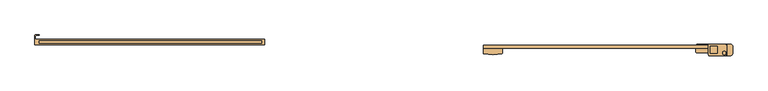
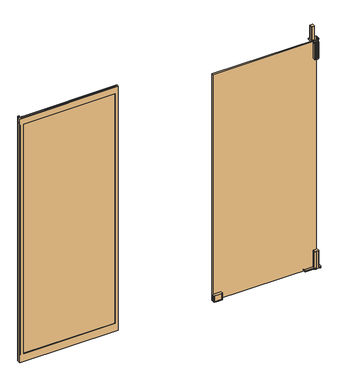
"""IFC4 building model written with IfcOpenShell, lengths in millimetres: door geometry, Otomatik Kapı-Tek Kanat : Otomatik Kapı - Tek Kanat."""

from ifc_helpers import new_model, si_unit, frame, origin, origin_with_axes, place, context, project, spatial, polyline, circle_curve, outline, extrude, source, transform, mapped, element, save
from ifc_brep_helpers import plane_surface, cylinder_surface, revolved_surface, advanced_brep


def door_efeaefdb(model_context):
    return source(origin(), model_context, "Body", "SolidModel", [
        advanced_brep(
        [(-802.5, -155.7669497, 8.0000212), (-799.5330503, -152.8, 8.0000212), (-787.49925, -152.8, 8.0000212), (-787.49925, -154.8, 8.0000212), (-799.4861454, -154.8, 8.0000212), (-800.5, -155.8138546, 8.0000212), (-800.5, -167.3, 8.0000212), (-2.5, -167.3000082, 8.0000212), (-2.5, -187.3, 8.0000212), (-802.5, -187.3, 8.0000212), (-787.49925, -180.7974169, 8.0000212), (-12.4985, -180.7974169, 8.0000212), (-12.4985, -173.8001834, 8.0000212), (-787.49925, -173.8001834, 8.0000212), (-800.5, -167.3, 2101.0), (-800.5, -155.8138546, 2101.0), (-799.4861454, -154.8, 2101.0), (-787.49925, -154.8, 2101.0), (-787.49925, -152.8, 2101.0), (-799.5330503, -152.8, 2101.0), (-802.5, -155.7669497, 2101.0), (-802.5, -187.3, 2101.0), (-2.5, -187.3, 2101.0), (-2.5, -167.3, 2101.0), (-787.49925, -172.299, 2101.0), (-12.4985, -172.299, 2101.0), (-12.4985, -182.301, 2101.0), (-787.49925, -182.301, 2101.0), (-802.5, -187.3, 78.000055), (-802.5, -185.3, 78.000055), (-802.5, -185.3, 62.9982446), (-802.5, -184.239458, 62.9982446), (-802.5, -184.239458, 2061.0007973), (-802.5, -185.3, 2061.0007973), (-802.5, -185.3, 2046.0007973), (-802.5, -187.3, 2046.0007973), (-772.4862373, -167.3, 2046.0004744), (-772.4862373, -169.2993721, 2046.0004744), (-772.4862373, -169.2993721, 77.9999799), (-772.4862373, -167.3, 77.9999799), (-787.49925, -169.2993721, 2061.0007973), (-787.49925, -169.2993721, 62.9982446), (-12.4985, -169.2993721, 62.9982446), (-12.4985, -169.2993721, 2061.0007973), (-27.4985, -169.2993721, 2046.0004744), (-27.4985, -169.2993721, 77.9999799), (-787.49925, -173.8001834, 33.4998483), (-787.49925, -180.7974169, 33.4998483), (-787.49925, -182.301, 2092.5), (-787.49925, -172.299, 2092.5), (-787.49925, -185.3, 2061.0007973), (-787.49925, -185.3, 62.9982446), (-802.3103756, -185.3, 78.000055), (-802.3103756, -185.3, 62.9982446), (-802.3103756, -185.3, 2061.0007973), (-802.3103756, -185.3, 2046.0007973), (-12.4985, -185.3, 2061.0007973), (-12.4985, -185.3, 62.9982446), (-772.4985, -185.3, 2046.0007973), (-772.4985, -185.3, 78.000055), (-27.4985, -185.3, 78.000055), (-27.4985, -185.3, 2046.0007973), (-772.4985, -187.3, 2046.0007973), (-772.4985, -187.3, 78.000055), (-799.439458, -187.3, 2046.0007973), (-799.439458, -187.3, 78.000055), (-27.4985, -187.3, 2046.0007973), (-27.4985, -187.3, 78.000055), (-27.4985, -167.3, 77.9999799), (-27.4985, -167.3, 2046.0004744), (-12.4985, -182.301, 2092.5), (-12.4985, -172.299, 2092.5), (-12.4985, -173.8001834, 33.4998483), (-12.4985, -180.7974169, 33.4998483)],
        [
            (0, 1, circle_curve(frame((-799.5330503, -155.7669497, 8.0000212), z_axis=(0.0, 0.0, -1.0), x_axis=(-1.0, 0.0, 0.0)), 2.9669497)),
            (1, 2),
            (2, 3),
            (3, 4),
            (4, 5, circle_curve(frame((-799.4861454, -155.8138546, 8.0000212), z_axis=(0.0, 0.0, 1.0), x_axis=(-1.0, 0.0, 0.0)), 1.0138546)),
            (5, 6),
            (6, 7),
            (7, 8),
            (8, 9),
            (9, 0),
            (10, 11),
            (11, 12),
            (12, 13),
            (13, 10),
            (14, 15),
            (15, 16, circle_curve(frame((-799.4861454, -155.8138546, 2101.0), z_axis=(0.0, 0.0, -1.0), x_axis=(-1.0, 0.0, 0.0)), 1.0138546)),
            (16, 17),
            (17, 18),
            (18, 19),
            (19, 20, circle_curve(frame((-799.5330503, -155.7669497, 2101.0), z_axis=(0.0, 0.0, 1.0), x_axis=(-1.0, 0.0, 0.0)), 2.9669497)),
            (20, 21),
            (21, 22),
            (22, 23),
            (23, 14),
            (24, 25),
            (25, 26),
            (26, 27),
            (27, 24),
            (20, 0),
            (9, 28),
            (28, 29),
            (29, 30),
            (30, 31),
            (31, 32),
            (32, 33),
            (33, 34),
            (34, 35),
            (35, 21),
            (1, 19),
            (18, 2),
            (17, 3),
            (36, 37),
            (37, 38),
            (38, 39),
            (39, 36),
            (40, 41),
            (41, 42),
            (42, 43),
            (43, 40),
            (37, 44),
            (44, 45),
            (45, 38),
            (13, 46),
            (46, 47),
            (47, 10),
            (27, 48),
            (48, 49),
            (49, 24),
            (40, 50),
            (50, 51),
            (51, 41),
            (29, 52),
            (52, 53),
            (53, 30),
            (33, 54),
            (54, 55),
            (55, 34),
            (50, 56),
            (56, 57),
            (57, 51),
            (58, 59),
            (59, 60),
            (60, 61),
            (61, 58),
            (58, 62),
            (62, 63),
            (63, 59),
            (35, 64),
            (64, 65),
            (65, 28),
            (8, 22),
            (62, 66),
            (66, 67),
            (67, 63),
            (23, 7),
            (6, 14),
            (39, 68),
            (68, 69),
            (69, 36),
            (16, 4),
            (5, 15),
            (54, 32, circle_curve(frame((-799.439458, -184.239458, 2061.0007973), z_axis=(0.0, 0.0, -1.0), x_axis=(-1.0, 0.0, 0.0)), 3.060542)),
            (31, 53, circle_curve(frame((-799.439458, -184.239458, 62.9982446), z_axis=(0.0, 0.0, 1.0), x_axis=(-1.0, 0.0, 0.0)), 3.060542)),
            (52, 65, circle_curve(frame((-799.439458, -184.239458, 78.000055), z_axis=(0.0, 0.0, 1.0), x_axis=(-1.0, 0.0, 0.0)), 3.060542)),
            (64, 55, circle_curve(frame((-799.439458, -184.239458, 2046.0007973), z_axis=(0.0, 0.0, -1.0), x_axis=(-1.0, 0.0, 0.0)), 3.060542)),
            (26, 70),
            (70, 48),
            (70, 71),
            (71, 49),
            (71, 25),
            (69, 44),
            (43, 56),
            (61, 66),
            (67, 60),
            (57, 42),
            (45, 68),
            (12, 72),
            (72, 46),
            (72, 73),
            (73, 47),
            (73, 11),
        ],
        [
            plane_surface(frame((-802.5, -167.3, 8.0000212), z_axis=(0.0, 0.0, -1.0), x_axis=(0.0, -1.0, 0.0))),
            plane_surface(frame((-802.5, -167.3, 2101.0), z_axis=(0.0, 0.0, 1.0), x_axis=(0.0, -1.0, 0.0))),
            plane_surface(frame((-802.5, -184.239458, 8.0000212), z_axis=(-1.0, 0.0, 0.0), x_axis=(0.0, 0.0, 1.0))),
            plane_surface(frame((-799.5330503, -152.8, 8.0000212), z_axis=(0.0, 1.0, 0.0), x_axis=(0.0, 0.0, 1.0))),
            plane_surface(frame((-787.49925, -152.8, 8.0000212), z_axis=(1.0, 0.0, 0.0), x_axis=(0.0, 0.0, 1.0))),
            plane_surface(frame((-772.4862373, -167.3, 8.0000212), z_axis=(1.0, 0.0, 0.0), x_axis=(0.0, 0.0, 1.0))),
            plane_surface(frame((-772.4862373, -169.2993721, 8.0000212), z_axis=(0.0, -1.0, 0.0), x_axis=(0.0, 0.0, 1.0))),
            plane_surface(frame((-787.49925, -169.2993721, 8.0000212), z_axis=(1.0, 0.0, 0.0), x_axis=(0.0, 0.0, 1.0))),
            plane_surface(frame((-787.49925, -185.3, 8.0000212), z_axis=(0.0, 1.0, 0.0), x_axis=(0.0, 0.0, 1.0))),
            plane_surface(frame((-772.4985, -185.3, 8.0000212), z_axis=(1.0, 0.0, 0.0), x_axis=(0.0, 0.0, 1.0))),
            plane_surface(frame((-772.4985, -187.3, 8.0000212), z_axis=(0.0, -1.0, 0.0), x_axis=(0.0, 0.0, 1.0))),
            plane_surface(frame((-800.5, -167.3, 8.0000212), z_axis=(0.0, 1.0, 0.0), x_axis=(0.0, 0.0, 1.0))),
            plane_surface(frame((-787.49925, -154.8, 8.0000212), z_axis=(0.0, -1.0, 0.0), x_axis=(0.0, 0.0, 1.0))),
            plane_surface(frame((-800.5, -155.8138546, 8.0000212), z_axis=(1.0, 0.0, 0.0), x_axis=(0.0, 0.0, 1.0))),
            cylinder_surface(frame((-799.439458, -184.239458, 8.0000212), z_axis=(0.0, 0.0, -1.0), x_axis=(-1.0, 0.0, 0.0)), 3.060542),
            cylinder_surface(frame((-799.5330503, -155.7669497, 8.0000212), z_axis=(0.0, 0.0, -1.0), x_axis=(-1.0, 0.0, 0.0)), 2.9669497),
            revolved_surface(polyline([(-800.5, -155.8138546, 2101.0), (-800.5, -155.8138546, 8.0000212)]), (-799.4861454, -155.8138546, 8.0000212), (0.0, 0.0, 1.0)),
            plane_surface(frame((-2.5, -167.3, 2101.0), z_axis=(1.0, 0.0, 0.0), x_axis=(0.0, -1.0, 0.0))),
            plane_surface(frame((-802.5, -182.301, 2101.0), z_axis=(0.0, 1.0, 0.0), x_axis=(1.0, 0.0, 0.0))),
            plane_surface(frame((-802.5, -182.301, 2092.5), z_axis=(0.0, 0.0, 1.0), x_axis=(1.0, 0.0, 0.0))),
            plane_surface(frame((-802.5, -172.299, 2092.5), z_axis=(0.0, -1.0, 0.0), x_axis=(1.0, 0.0, 0.0))),
            plane_surface(frame((-802.5, -167.3, 2046.0004744), z_axis=(0.0, 0.0, -1.0), x_axis=(1.0, 0.0, 0.0))),
            plane_surface(frame((-802.5, -169.3, 2061.0007973), z_axis=(0.0, 0.0, -1.0), x_axis=(1.0, 0.0, 0.0))),
            plane_surface(frame((-802.5, -185.3, 2046.0007973), z_axis=(0.0, 0.0, -1.0), x_axis=(1.0, 0.0, 0.0))),
            plane_surface(frame((-802.5, -187.3, 78.000055), z_axis=(0.0, 0.0, 1.0), x_axis=(1.0, 0.0, 0.0))),
            plane_surface(frame((-802.5, -185.3, 62.9982446), z_axis=(0.0, 0.0, 1.0), x_axis=(1.0, 0.0, 0.0))),
            plane_surface(frame((-802.5, -169.3000224, 77.9999799), z_axis=(0.0, 0.0, 1.0), x_axis=(1.0, 0.0, 0.0))),
            plane_surface(frame((-802.5, -173.8001834, 8.0000212), z_axis=(0.0, -1.0, 0.0), x_axis=(1.0, 0.0, 0.0))),
            plane_surface(frame((-802.5, -173.8001834, 33.4998483), z_axis=(0.0, 0.0, -1.0), x_axis=(1.0, 0.0, 0.0))),
            plane_surface(frame((-802.5, -180.7974169, 33.4998483), z_axis=(0.0, 1.0, 0.0), x_axis=(1.0, 0.0, 0.0))),
            plane_surface(frame((-27.4985, -187.3, 8.0000212), z_axis=(-1.0, 0.0, 0.0), x_axis=(0.0, 0.0, 1.0))),
            plane_surface(frame((-12.4985, -185.3, 8.0000212), z_axis=(-1.0, 0.0, 0.0), x_axis=(0.0, 0.0, 1.0))),
            plane_surface(frame((-27.4985, -169.3, 8.0000212), z_axis=(-1.0, 0.0, 0.0), x_axis=(0.0, 0.0, 1.0))),
        ],
        [
            (0, [[1, 2, 3, 4, 5, 6, 7, 8, 9, 10], [11, 12, 13, 14]]),
            (1, [[15, 16, 17, 18, 19, 20, 21, 22, 23, 24], [25, 26, 27, 28]]),
            (2, [[29, -10, 30, 31, 32, 33, 34, 35, 36, 37, 38, -21]]),
            (3, [[-2, 39, -19, 40]]),
            (4, [[-3, -40, -18, 41]]),
            (5, [[42, 43, 44, 45]]),
            (6, [[46, 47, 48, 49], [-43, 50, 51, 52]]),
            (7, [[-14, 53, 54, 55]]),
            (7, [[-28, 56, 57, 58]]),
            (7, [[59, 60, 61, -46]]),
            (8, [[-32, 62, 63, 64]]),
            (8, [[-36, 65, 66, 67]]),
            (8, [[-60, 68, 69, 70], [71, 72, 73, 74]]),
            (9, [[75, 76, 77, -71]]),
            (10, [[-22, -38, 78, 79, 80, -30, -9, 81], [82, 83, 84, -76]]),
            (11, [[-24, 85, -7, 86], [87, 88, 89, -45]]),
            (12, [[-4, -41, -17, 90]]),
            (13, [[-6, 91, -15, -86]]),
            (14, [[92, -34, 93, -63, 94, -79, 95, -66]]),
            (15, [[-1, -29, -20, -39]]),
            (16, [[-5, -90, -16, -91]]),
            (17, [[-81, -8, -85, -23]]),
            (18, [[-56, -27, 96, 97]]),
            (19, [[-57, -97, 98, 99]]),
            (20, [[-58, -99, 100, -25]]),
            (21, [[-42, -89, 101, -50]]),
            (22, [[-35, -92, -65]]),
            (22, [[-68, -59, -49, 102]]),
            (23, [[-37, -67, -95, -78]]),
            (23, [[-75, -74, 103, -82]]),
            (24, [[-31, -80, -94, -62]]),
            (24, [[-77, -84, 104, -72]]),
            (25, [[-33, -64, -93]]),
            (25, [[-47, -61, -70, 105]]),
            (26, [[-44, -52, 106, -87]]),
            (27, [[-53, -13, 107, 108]]),
            (28, [[-54, -108, 109, 110]]),
            (29, [[-55, -110, 111, -11]]),
            (30, [[-73, -104, -83, -103]]),
            (31, [[-12, -111, -109, -107]]),
            (31, [[-26, -100, -98, -96]]),
            (31, [[-69, -102, -48, -105]]),
            (32, [[-88, -106, -51, -101]]),
        ],
    ),
        extrude(outline(polyline([(-14.9985, -170.3000147), (-14.9985, -180.2993696), (-784.0, -180.2993696), (-784.0, -170.3000147), (-14.9985, -170.3000147)])), frame((0.0, 0.0, 65.4907153), z_axis=(0.0, 0.0, 1.0), x_axis=(1.0, 0.0, 0.0)), (0.0, 0.0, 1.0), 1993.010082),
        extrude(outline(polyline([(-170.3000393, 2058.9584681), (-170.3000367, 2075.4578872), (-169.3000368, 2075.4578872), (-169.3000392, 2060.1996761), (-167.7000392, 2060.1994116), (-167.7000392, 2059.1856312), (-170.3000393, 2058.9584681)])), frame((-802.5, 0.0, 0.0), z_axis=(1.0, 0.0, 0.0), x_axis=(0.0, 1.0, 0.0)), (0.0, 0.0, 1.0), 800.0),
        extrude(outline(polyline([(-170.3000147, 79.2411881), (-167.7000146, 79.0140251), (-167.7000146, 78.0002446), (-169.3000145, 77.9999802), (-169.3000145, 62.7412326), (-170.3000121, 62.7417691), (-170.3000147, 79.2411881)])), frame((-802.5, 0.0, 0.0), z_axis=(1.0, 0.0, 0.0), x_axis=(0.0, 1.0, 0.0)), (0.0, 0.0, 1.0), 800.0),
        extrude(outline(polyline([(-783.1860852, -169.2999998), (-772.5, -169.2999998), (-772.5, -167.6999998), (-771.385912, -167.6999998), (-771.0906874, -170.50022), (-783.1860852, -170.50022), (-783.1860852, -169.2999998)])), frame((0.0, 0.0, 8.0000212), z_axis=(0.0, 0.0, 1.0), x_axis=(1.0, 0.0, 0.0)), (0.0, 0.0, 1.0), 2092.9999788),
        advanced_brep(
        [(1574.3473639, -189.1450647, 150.5), (1599.9937802, -189.1450647, 150.5), (1599.9937802, -199.1283088, 150.5), (1574.9937802, -199.1283088, 150.5), (1574.9937802, -217.3610561, 150.5), (1587.4005623, -224.1450647, 150.5), (1605.2100763, -224.1450647, 150.5), (1606.9937802, -222.3613608, 150.5), (1606.9937802, -187.0776187, 150.5), (1605.0612263, -185.1450647, 150.5), (1576.2799178, -185.1450647, 150.5), (1574.3473639, -187.0776187, 150.5), (1578.9203726, -221.1098306, 8.0), (1574.9937802, -217.3610561, 8.0), (1577.1630779, -219.3712473, 8.0), (1574.3473639, -189.1450647, 8.0), (1599.9937802, -189.1450647, 8.0), (1599.9937802, -199.1283088, 8.0), (1574.9937802, -199.1283088, 8.0), (1587.4005623, -224.1450647, 8.0), (1587.4005623, -224.1450647, 0.0), (1619.8416735, -224.1450647, 0.0), (1619.8416735, -224.1450647, 8.0), (1605.2100763, -224.1450647, 8.0), (1606.9937802, -222.3613608, 8.0), (1606.9937802, -187.0776187, 8.0), (1605.0612263, -185.1450647, 8.0), (1619.9440671, -185.1450647, 8.0), (1619.9440671, -185.1450647, 0.0), (1504.0, -185.1450647, 0.0), (1504.0, -185.1450647, 8.0), (1576.2799178, -185.1450647, 8.0), (1574.3473639, -187.0776187, 8.0), (1627.0, -192.2009976, 0.0), (1627.0, -216.9867382, 0.0), (1577.1630779, -219.3712473, 0.0), (1568.1, -215.1450647, 0.0), (1504.0, -215.1450647, 0.0), (1499.0, -210.1450647, 0.0), (1499.0, -190.1450647, 0.0), (1627.0, -216.9867382, 8.0), (1627.0, -192.2009976, 8.0), (1499.0, -190.1450647, 8.0), (1499.0, -210.1450647, 8.0), (1504.0, -215.1450647, 8.0), (1568.1, -215.1450647, 8.0)],
        [
            (0, 1),
            (1, 2),
            (2, 3),
            (3, 4),
            (4, 5, circle_curve(frame((1588.8230743, -206.8065986, 150.5), z_axis=(0.0, 0.0, 1.0), x_axis=(-1.0, 0.0, 0.0)), 17.3967223)),
            (5, 6),
            (6, 7, circle_curve(frame((1605.2100763, -222.3613608, 150.5), z_axis=(0.0, 0.0, 1.0), x_axis=(-1.0, 0.0, 0.0)), 1.7837039)),
            (7, 8),
            (8, 9, circle_curve(frame((1605.0612263, -187.0776187, 150.5), z_axis=(0.0, 0.0, 1.0), x_axis=(-1.0, 0.0, 0.0)), 1.932554)),
            (9, 10),
            (10, 11, circle_curve(frame((1576.2799178, -187.0776187, 150.5), z_axis=(0.0, 0.0, 1.0), x_axis=(-1.0, 0.0, 0.0)), 1.932554)),
            (11, 0),
            (12, 13, circle_curve(frame((1588.8230743, -206.8065986, 8.0), z_axis=(0.0, 0.0, -1.0), x_axis=(-1.0, 0.0, 0.0)), 17.3967223)),
            (13, 14, circle_curve(frame((1568.1, -226.9760726, 8.0), z_axis=(0.0, 0.0, -1.0), x_axis=(-1.0, 0.0, 0.0)), 11.8310079)),
            (14, 12, circle_curve(frame((1587.4005623, -210.7809779, 8.0), z_axis=(0.0, 0.0, 1.0), x_axis=(-1.0, 0.0, 0.0)), 13.3640868)),
            (0, 15),
            (15, 16),
            (16, 1),
            (16, 17),
            (17, 2),
            (17, 18),
            (18, 3),
            (18, 13),
            (13, 4),
            (12, 19, circle_curve(frame((1588.8230743, -206.8065986, 8.0), z_axis=(0.0, 0.0, 1.0), x_axis=(-1.0, 0.0, 0.0)), 17.3967223)),
            (19, 5),
            (19, 20),
            (20, 21),
            (21, 22),
            (22, 23),
            (23, 6),
            (23, 24, circle_curve(frame((1605.2100763, -222.3613608, 8.0), z_axis=(0.0, 0.0, 1.0), x_axis=(-1.0, 0.0, 0.0)), 1.7837039)),
            (24, 7),
            (24, 25),
            (25, 8),
            (25, 26, circle_curve(frame((1605.0612263, -187.0776187, 8.0), z_axis=(0.0, 0.0, 1.0), x_axis=(-1.0, 0.0, 0.0)), 1.932554)),
            (26, 9),
            (26, 27),
            (27, 28),
            (28, 29),
            (29, 30),
            (30, 31),
            (31, 10),
            (31, 32, circle_curve(frame((1576.2799178, -187.0776187, 8.0), z_axis=(0.0, 0.0, 1.0), x_axis=(-1.0, 0.0, 0.0)), 1.932554)),
            (32, 11),
            (32, 15),
            (28, 33, circle_curve(frame((1619.9440671, -192.2009976, 0.0), z_axis=(0.0, 0.0, -1.0), x_axis=(-1.0, 0.0, 0.0)), 7.0559329)),
            (33, 34),
            (34, 21, circle_curve(frame((1619.8416735, -216.9867382, 0.0), z_axis=(0.0, 0.0, -1.0), x_axis=(-1.0, 0.0, 0.0)), 7.1583265)),
            (20, 35, circle_curve(frame((1587.4005623, -210.7809779, 0.0), z_axis=(0.0, 0.0, -1.0), x_axis=(-1.0, 0.0, 0.0)), 13.3640868)),
            (35, 36, circle_curve(frame((1568.1, -226.9760726, 0.0), z_axis=(0.0, 0.0, 1.0), x_axis=(-1.0, 0.0, 0.0)), 11.8310079)),
            (36, 37),
            (37, 38, circle_curve(frame((1504.0, -210.1450647, 0.0), z_axis=(0.0, 0.0, -1.0), x_axis=(-1.0, 0.0, 0.0)), 5.0)),
            (38, 39),
            (39, 29, circle_curve(frame((1504.0, -190.1450647, 0.0), z_axis=(0.0, 0.0, -1.0), x_axis=(-1.0, 0.0, 0.0)), 5.0)),
            (12, 19, circle_curve(frame((1587.4005623, -210.7809779, 8.0), z_axis=(0.0, 0.0, 1.0), x_axis=(-1.0, 0.0, 0.0)), 13.3640868)),
            (22, 40, circle_curve(frame((1619.8416735, -216.9867382, 8.0), z_axis=(0.0, 0.0, 1.0), x_axis=(-1.0, 0.0, 0.0)), 7.1583265)),
            (40, 41),
            (41, 27, circle_curve(frame((1619.9440671, -192.2009976, 8.0), z_axis=(0.0, 0.0, 1.0), x_axis=(-1.0, 0.0, 0.0)), 7.0559329)),
            (30, 42, circle_curve(frame((1504.0, -190.1450647, 8.0), z_axis=(0.0, 0.0, 1.0), x_axis=(-1.0, 0.0, 0.0)), 5.0)),
            (42, 43),
            (43, 44, circle_curve(frame((1504.0, -210.1450647, 8.0), z_axis=(0.0, 0.0, 1.0), x_axis=(-1.0, 0.0, 0.0)), 5.0)),
            (44, 45),
            (45, 13, circle_curve(frame((1568.1, -226.9760726, 8.0), z_axis=(0.0, 0.0, -1.0), x_axis=(-1.0, 0.0, 0.0)), 11.8310079)),
            (41, 33),
            (40, 34),
            (14, 35),
            (45, 36),
            (44, 37),
            (43, 38),
            (42, 39),
        ],
        [
            plane_surface(frame((1627.0, -185.1450647, 150.5), z_axis=(0.0, 0.0, 1.0), x_axis=(0.0, 1.0, 0.0))),
            plane_surface(frame((1627.0, -185.1450647, 8.0), z_axis=(0.0, 0.0, -1.0), x_axis=(0.0, 1.0, 0.0))),
            plane_surface(frame((1574.3473639, -189.1450647, 150.5), z_axis=(0.0, -1.0, 0.0), x_axis=(0.0, 0.0, -1.0))),
            plane_surface(frame((1599.9937802, -189.1450647, 150.5), z_axis=(-1.0, 0.0, 0.0), x_axis=(0.0, 0.0, -1.0))),
            plane_surface(frame((1599.9937802, -199.1283088, 150.5), z_axis=(0.0, 1.0, 0.0), x_axis=(0.0, 0.0, -1.0))),
            plane_surface(frame((1574.9937802, -199.1283088, 150.5), z_axis=(-1.0, 0.0, 0.0), x_axis=(0.0, 0.0, -1.0))),
            cylinder_surface(frame((1588.8230743, -206.8065986, 150.5), z_axis=(0.0, 0.0, 1.0), x_axis=(-1.0, 0.0, 0.0)), 17.3967223),
            plane_surface(frame((1587.4005623, -224.1450647, 150.5), z_axis=(0.0, -1.0, 0.0), x_axis=(0.0, 0.0, -1.0))),
            cylinder_surface(frame((1605.2100763, -222.3613608, 150.5), z_axis=(0.0, 0.0, 1.0), x_axis=(-1.0, 0.0, 0.0)), 1.7837039),
            plane_surface(frame((1606.9937802, -222.3613608, 150.5), z_axis=(1.0, 0.0, 0.0), x_axis=(0.0, 0.0, -1.0))),
            cylinder_surface(frame((1605.0612263, -187.0776187, 150.5), z_axis=(0.0, 0.0, 1.0), x_axis=(-1.0, 0.0, 0.0)), 1.932554),
            plane_surface(frame((1605.0612263, -185.1450647, 150.5), z_axis=(0.0, 1.0, 0.0), x_axis=(0.0, 0.0, -1.0))),
            cylinder_surface(frame((1576.2799178, -187.0776187, 150.5), z_axis=(0.0, 0.0, 1.0), x_axis=(-1.0, 0.0, 0.0)), 1.932554),
            plane_surface(frame((1574.3473639, -187.0776187, 150.5), z_axis=(-1.0, 0.0, 0.0), x_axis=(0.0, 0.0, -1.0))),
            plane_surface(frame((1627.0, -185.1450647, 0.0), z_axis=(0.0, 0.0, -1.0), x_axis=(0.0, 1.0, 0.0))),
            plane_surface(frame((1627.0, -185.1450647, 8.0), z_axis=(0.0, 0.0, 1.0), x_axis=(0.0, 1.0, 0.0))),
            cylinder_surface(frame((1619.9440671, -192.2009976, 0.0), z_axis=(0.0, 0.0, -1.0), x_axis=(-1.0, 0.0, 0.0)), 7.0559329),
            plane_surface(frame((1627.0, -192.2009976, 0.0), z_axis=(1.0, 0.0, 0.0), x_axis=(0.0, 0.0, 1.0))),
            cylinder_surface(frame((1619.8416735, -216.9867382, 0.0), z_axis=(0.0, 0.0, -1.0), x_axis=(-1.0, 0.0, 0.0)), 7.1583265),
            cylinder_surface(frame((1587.4005623, -210.7809779, 0.0), z_axis=(0.0, 0.0, -1.0), x_axis=(-1.0, 0.0, 0.0)), 13.3640868),
            revolved_surface(polyline([(1556.2689920999999, -226.9760726, 8.0), (1556.2689920999999, -226.9760726, 0.0)]), (1568.1, -226.9760726, 0.0), (0.0, 0.0, 1.0)),
            plane_surface(frame((1568.1, -215.1450647, 0.0), z_axis=(0.0, -1.0, 0.0), x_axis=(0.0, 0.0, 1.0))),
            cylinder_surface(frame((1504.0, -210.1450647, 0.0), z_axis=(0.0, 0.0, -1.0), x_axis=(-1.0, 0.0, 0.0)), 5.0),
            plane_surface(frame((1499.0, -210.1450647, 0.0), z_axis=(-1.0, 0.0, 0.0), x_axis=(0.0, 0.0, 1.0))),
            cylinder_surface(frame((1504.0, -190.1450647, 0.0), z_axis=(0.0, 0.0, -1.0), x_axis=(-1.0, 0.0, 0.0)), 5.0),
        ],
        [
            (0, [[1, 2, 3, 4, 5, 6, 7, 8, 9, 10, 11, 12]]),
            (1, [[13, 14, 15]]),
            (2, [[-1, 16, 17, 18]]),
            (3, [[-2, -18, 19, 20]]),
            (4, [[-3, -20, 21, 22]]),
            (5, [[-4, -22, 23, 24]]),
            (6, [[-5, -24, -13, 25, 26]]),
            (7, [[-6, -26, 27, 28, 29, 30, 31]]),
            (8, [[-7, -31, 32, 33]]),
            (9, [[-8, -33, 34, 35]]),
            (10, [[-9, -35, 36, 37]]),
            (11, [[-10, -37, 38, 39, 40, 41, 42, 43]]),
            (12, [[-11, -43, 44, 45]]),
            (13, [[-12, -45, 46, -16]]),
            (14, [[-40, 47, 48, 49, -28, 50, 51, 52, 53, 54, 55]]),
            (15, [[56, -25]]),
            (15, [[57, 58, 59, -38, -36, -34, -32, -30]]),
            (15, [[60, 61, 62, 63, 64, -23, -21, -19, -17, -46, -44, -42]]),
            (16, [[-47, -39, -59, 65]]),
            (17, [[-48, -65, -58, 66]]),
            (18, [[-49, -66, -57, -29]]),
            (19, [[-50, -27, -56, -15, 67]]),
            (20, [[-51, -67, -14, -64, 68]]),
            (21, [[-52, -68, -63, 69]]),
            (22, [[-53, -69, -62, 70]]),
            (23, [[-54, -70, -61, 71]]),
            (24, [[-55, -71, -60, -41]]),
        ],
    ),
        advanced_brep(
        [(1572.1438552, -192.4241594, 2085.0), (1550.8144257, -192.4241594, 2085.0), (1548.9791404, -194.2594446, 2085.0), (1548.9791404, -215.5888742, 2085.0), (1550.8144257, -217.4241594, 2085.0), (1572.1438552, -217.4241594, 2085.0), (1573.9791404, -215.5888742, 2085.0), (1573.9791404, -194.2594446, 2085.0), (1572.1438552, -192.4241594, 1970.0), (1550.8144257, -192.4241594, 1970.0), (1548.9791404, -194.2594446, 1970.0), (1548.9791404, -215.5888742, 1970.0), (1550.8144257, -217.4241594, 1970.0), (1572.1438552, -217.4241594, 1970.0), (1573.9791404, -215.5888742, 1970.0), (1573.9791404, -194.2594446, 1970.0), (1545.9964024, -185.1450647, 1970.0), (1542.9937802, -188.1476868, 1970.0), (1542.9937802, -221.823489, 1970.0), (1546.3153559, -225.1450647, 1970.0), (1597.9937802, -225.1450647, 1970.0), (1606.9937802, -216.1450647, 1970.0), (1606.9937802, -193.9739051, 1970.0), (1598.1649399, -185.1450647, 1970.0), (1597.9937802, -222.0450647, 1970.0), (1597.9937802, -210.2450647, 1970.0), (1545.9964024, -185.1450647, 1964.0), (1598.1649399, -185.1450647, 1964.0), (1606.9937802, -193.9739051, 1964.0), (1606.9937802, -216.1450647, 1964.0), (1597.9937802, -225.1450647, 1964.0), (1546.3153559, -225.1450647, 1964.0), (1542.9937802, -221.823489, 1964.0), (1542.9937802, -188.1476868, 1964.0), (1597.9937802, -210.2450647, 1964.0), (1597.9937802, -222.0450647, 1964.0), (1606.9937802, -216.1450647, 1798.2), (1591.4461955, -222.319944, 1798.2), (1587.411505, -225.1450647, 1798.2), (1578.0937802, -225.1450647, 1798.2), (1574.9937802, -222.0450647, 1798.2), (1574.9937802, -199.2450647, 1798.2), (1599.7937802, -199.2450647, 1798.2), (1599.7937802, -189.2450647, 1798.2), (1574.9937802, -189.2450647, 1798.2), (1574.9937802, -186.4710526, 1798.2), (1576.3197681, -185.1450647, 1798.2), (1605.7821796, -185.1450647, 1798.2), (1606.9937802, -186.3566653, 1798.2), (1587.2194224, -210.2450647, 1798.2), (1578.0937802, -210.2450647, 1798.2), (1578.0937802, -221.0562868, 1798.2), (1579.0825581, -222.0450647, 1798.2), (1587.1673699, -222.0450647, 1798.2), (1588.942968, -219.8725331, 1798.2), (1588.9937802, -212.0194225, 1798.2), (1597.9937802, -210.2450647, 1798.2), (1597.9937802, -222.0450647, 1798.2), (1606.9937802, -216.1450647, 1943.2), (1606.9937802, -186.3566653, 1943.2), (1605.7821796, -185.1450647, 1943.2), (1576.3197681, -185.1450647, 1943.2), (1574.9937802, -186.4710526, 1943.2), (1574.9937802, -189.2450647, 1943.2), (1599.7937802, -189.2450647, 1943.2), (1599.7937802, -199.2450647, 1943.2), (1574.9937802, -199.2450647, 1943.2), (1574.9937802, -209.0670845, 1943.2), (1576.1717604, -210.2450647, 1943.2), (1587.2194224, -210.2450647, 1943.2), (1588.9937802, -212.0194225, 1943.2), (1588.9937802, -216.1450647, 1943.2), (1597.9937802, -222.0450647, 1943.2), (1597.9937802, -210.2450647, 1943.2), (1574.9937802, -222.0450647, 1933.2), (1574.9937802, -209.0670845, 1933.2), (1576.1717604, -210.2450647, 1933.2), (1578.0937802, -210.2450647, 1933.2), (1588.9937802, -219.8725331, 1933.2), (1588.9937802, -216.1450647, 1933.2), (1591.4461955, -222.319944, 1933.2), (1597.9937802, -222.0450647, 1943.2), (1597.9937802, -210.2450647, 1943.2), (1578.0937802, -225.1450647, 1933.2), (1587.411505, -225.1450647, 1933.2), (1587.1673699, -222.0450647, 1933.2), (1579.0825581, -222.0450647, 1933.2), (1578.0937802, -221.0562868, 1933.2), (1597.9937802, -210.2450647, 1976.5286826), (1597.9937802, -222.0450647, 1976.5286826)],
        [
            (0, 1),
            (1, 2, circle_curve(frame((1550.8144257, -194.2594446, 2085.0), z_axis=(0.0, 0.0, 1.0), x_axis=(0.0, -1.0, 0.0)), 1.8352852)),
            (2, 3),
            (3, 4, circle_curve(frame((1550.8144257, -215.5888742, 2085.0), z_axis=(0.0, 0.0, 1.0), x_axis=(0.0, 1.0, 0.0)), 1.8352852)),
            (4, 5),
            (5, 6, circle_curve(frame((1572.1438552, -215.5888742, 2085.0), z_axis=(0.0, 0.0, 1.0), x_axis=(0.0, 1.0, 0.0)), 1.8352852)),
            (6, 7),
            (7, 0, circle_curve(frame((1572.1438552, -194.2594446, 2085.0), z_axis=(0.0, 0.0, 1.0), x_axis=(0.0, -1.0, 0.0)), 1.8352852)),
            (0, 8),
            (8, 9),
            (9, 1),
            (9, 10, circle_curve(frame((1550.8144257, -194.2594446, 1970.0), z_axis=(0.0, 0.0, 1.0), x_axis=(0.0, -1.0, 0.0)), 1.8352852)),
            (10, 2),
            (10, 11),
            (11, 3),
            (11, 12, circle_curve(frame((1550.8144257, -215.5888742, 1970.0), z_axis=(0.0, 0.0, 1.0), x_axis=(0.0, 1.0, 0.0)), 1.8352852)),
            (12, 4),
            (12, 13),
            (13, 5),
            (13, 14, circle_curve(frame((1572.1438552, -215.5888742, 1970.0), z_axis=(0.0, 0.0, 1.0), x_axis=(0.0, 1.0, 0.0)), 1.8352852)),
            (14, 6),
            (14, 15),
            (15, 7),
            (15, 8, circle_curve(frame((1572.1438552, -194.2594446, 1970.0), z_axis=(0.0, 0.0, 1.0), x_axis=(0.0, -1.0, 0.0)), 1.8352852)),
            (16, 17, circle_curve(frame((1545.9964024, -188.1476868, 1970.0), z_axis=(0.0, 0.0, 1.0), x_axis=(0.0, -1.0, 0.0)), 3.0026222)),
            (17, 18),
            (18, 19, circle_curve(frame((1546.3153559, -221.823489, 1970.0), z_axis=(0.0, 0.0, 1.0), x_axis=(0.0, -1.0, 0.0)), 3.3215757)),
            (19, 20),
            (20, 21, circle_curve(frame((1597.9937802, -216.1450647, 1970.0), z_axis=(0.0, 0.0, 1.0), x_axis=(0.0, -1.0, 0.0)), 9.0)),
            (21, 22),
            (22, 23, circle_curve(frame((1598.1649399, -193.9739051, 1970.0), z_axis=(0.0, 0.0, 1.0), x_axis=(0.0, -1.0, 0.0)), 8.8288404)),
            (23, 16),
            (24, 25, circle_curve(frame((1597.9937802, -216.1450647, 1970.0), z_axis=(0.0, 0.0, -1.0), x_axis=(0.0, -1.0, 0.0)), 5.9)),
            (25, 24, circle_curve(frame((1597.9937802, -216.1450647, 1970.0), z_axis=(0.0, 0.0, -1.0), x_axis=(0.0, -1.0, 0.0)), 5.9)),
            (26, 27),
            (27, 28, circle_curve(frame((1598.1649399, -193.9739051, 1964.0), z_axis=(0.0, 0.0, -1.0), x_axis=(0.0, -1.0, 0.0)), 8.8288404)),
            (28, 29),
            (29, 30, circle_curve(frame((1597.9937802, -216.1450647, 1964.0), z_axis=(0.0, 0.0, -1.0), x_axis=(0.0, -1.0, 0.0)), 9.0)),
            (30, 31),
            (31, 32, circle_curve(frame((1546.3153559, -221.823489, 1964.0), z_axis=(0.0, 0.0, -1.0), x_axis=(0.0, -1.0, 0.0)), 3.3215757)),
            (32, 33),
            (33, 26, circle_curve(frame((1545.9964024, -188.1476868, 1964.0), z_axis=(0.0, 0.0, -1.0), x_axis=(0.0, -1.0, 0.0)), 3.0026222)),
            (34, 35, circle_curve(frame((1597.9937802, -216.1450647, 1964.0), z_axis=(0.0, 0.0, 1.0), x_axis=(0.0, -1.0, 0.0)), 5.9)),
            (35, 34, circle_curve(frame((1597.9937802, -216.1450647, 1964.0), z_axis=(0.0, 0.0, 1.0), x_axis=(0.0, -1.0, 0.0)), 5.9)),
            (23, 27),
            (26, 16),
            (22, 28),
            (21, 29),
            (20, 30),
            (19, 31),
            (18, 32),
            (17, 33),
            (36, 37, circle_curve(frame((1597.9937802, -216.1450647, 1798.2), z_axis=(0.0, 0.0, -1.0), x_axis=(0.0, -1.0, 0.0)), 9.0)),
            (37, 38, circle_curve(frame((1586.7260693, -219.8725331, 1798.2), z_axis=(0.0, 0.0, -1.0), x_axis=(0.0, -1.0, 0.0)), 5.3168987)),
            (38, 39),
            (39, 40, circle_curve(frame((1578.0937802, -222.0450647, 1798.2), z_axis=(0.0, 0.0, -1.0), x_axis=(0.0, -1.0, 0.0)), 3.1)),
            (40, 41),
            (41, 42),
            (42, 43),
            (43, 44),
            (44, 45),
            (45, 46, circle_curve(frame((1576.3197681, -186.4710526, 1798.2), z_axis=(0.0, 0.0, -1.0), x_axis=(0.0, -1.0, 0.0)), 1.3259879)),
            (46, 47),
            (47, 48, circle_curve(frame((1605.7821796, -186.3566653, 1798.2), z_axis=(0.0, 0.0, -1.0), x_axis=(0.0, -1.0, 0.0)), 1.2116006)),
            (48, 36),
            (49, 50),
            (50, 51),
            (51, 52, circle_curve(frame((1579.0825581, -221.0562868, 1798.2), z_axis=(0.0, 0.0, 1.0), x_axis=(0.0, -1.0, 0.0)), 0.9887779)),
            (52, 53),
            (53, 54, circle_curve(frame((1586.7260693, -219.8725331, 1798.2), z_axis=(0.0, 0.0, 1.0), x_axis=(0.0, -1.0, 0.0)), 2.2168987)),
            (54, 55),
            (55, 49, circle_curve(frame((1587.2194224, -212.0194225, 1798.2), z_axis=(0.0, 0.0, 1.0), x_axis=(0.0, -1.0, 0.0)), 1.7743579)),
            (56, 57, circle_curve(frame((1597.9937802, -216.1450647, 1798.2), z_axis=(0.0, 0.0, 1.0), x_axis=(0.0, -1.0, 0.0)), 5.9)),
            (57, 56, circle_curve(frame((1597.9937802, -216.1450647, 1798.2), z_axis=(0.0, 0.0, 1.0), x_axis=(0.0, -1.0, 0.0)), 5.9)),
            (58, 59),
            (59, 60, circle_curve(frame((1605.7821796, -186.3566653, 1943.2), z_axis=(0.0, 0.0, 1.0), x_axis=(0.0, -1.0, 0.0)), 1.2116006)),
            (60, 61),
            (61, 62, circle_curve(frame((1576.3197681, -186.4710526, 1943.2), z_axis=(0.0, 0.0, 1.0), x_axis=(0.0, -1.0, 0.0)), 1.3259879)),
            (62, 63),
            (63, 64),
            (64, 65),
            (65, 66),
            (66, 67),
            (67, 68, circle_curve(frame((1576.1717604, -209.0670845, 1943.2), z_axis=(0.0, 0.0, 1.0), x_axis=(0.0, -1.0, 0.0)), 1.1779802)),
            (68, 69),
            (69, 70, circle_curve(frame((1587.2194224, -212.0194225, 1943.2), z_axis=(0.0, 0.0, -1.0), x_axis=(0.0, -1.0, 0.0)), 1.7743579)),
            (70, 71),
            (71, 58, circle_curve(frame((1597.9937802, -216.1450647, 1943.2), z_axis=(0.0, 0.0, 1.0), x_axis=(0.0, -1.0, 0.0)), 9.0)),
            (72, 73, circle_curve(frame((1597.9937802, -216.1450647, 1943.2), z_axis=(0.0, 0.0, -1.0), x_axis=(0.0, -1.0, 0.0)), 5.9)),
            (73, 72, circle_curve(frame((1597.9937802, -216.1450647, 1943.2), z_axis=(0.0, 0.0, -1.0), x_axis=(0.0, -1.0, 0.0)), 5.9)),
            (48, 59),
            (58, 36),
            (47, 60),
            (46, 61),
            (45, 62),
            (44, 63),
            (43, 64),
            (42, 65),
            (41, 66),
            (40, 74),
            (74, 75),
            (75, 67),
            (75, 76, circle_curve(frame((1576.1717604, -209.0670845, 1933.2), z_axis=(0.0, 0.0, 1.0), x_axis=(0.0, -1.0, 0.0)), 1.1779802)),
            (76, 68),
            (76, 77),
            (77, 50),
            (49, 69),
            (55, 70),
            (54, 78),
            (78, 79),
            (79, 71),
            (79, 80, circle_curve(frame((1597.9937802, -216.1450647, 1933.2), z_axis=(0.0, 0.0, 1.0), x_axis=(0.0, -1.0, 0.0)), 9.0)),
            (80, 37),
            (57, 81),
            (81, 82, circle_curve(frame((1597.9937802, -216.1450647, 1943.2), z_axis=(0.0, 0.0, 1.0), x_axis=(0.0, -1.0, 0.0)), 5.9)),
            (82, 56),
            (82, 81, circle_curve(frame((1597.9937802, -216.1450647, 1943.2), z_axis=(0.0, 0.0, 1.0), x_axis=(0.0, -1.0, 0.0)), 5.9)),
            (83, 84),
            (84, 80, circle_curve(frame((1586.7260693, -219.8725331, 1933.2), z_axis=(0.0, 0.0, 1.0), x_axis=(0.0, -1.0, 0.0)), 5.3168987)),
            (78, 85, circle_curve(frame((1586.7260693, -219.8725331, 1933.2), z_axis=(0.0, 0.0, -1.0), x_axis=(0.0, -1.0, 0.0)), 2.2168987)),
            (85, 86),
            (86, 87, circle_curve(frame((1579.0825581, -221.0562868, 1933.2), z_axis=(0.0, 0.0, -1.0), x_axis=(0.0, -1.0, 0.0)), 0.9887779)),
            (87, 77),
            (74, 83, circle_curve(frame((1578.0937802, -222.0450647, 1933.2), z_axis=(0.0, 0.0, 1.0), x_axis=(0.0, -1.0, 0.0)), 3.1)),
            (39, 83),
            (87, 51),
            (86, 52),
            (85, 53),
            (84, 38),
            (88, 89, circle_curve(frame((1597.9937802, -216.1450647, 1976.5286826), z_axis=(0.0, 0.0, 1.0), x_axis=(0.0, -1.0, 0.0)), 5.9)),
            (89, 88, circle_curve(frame((1597.9937802, -216.1450647, 1976.5286826), z_axis=(0.0, 0.0, 1.0), x_axis=(0.0, -1.0, 0.0)), 5.9)),
            (35, 72),
            (73, 34),
            (89, 24),
            (25, 88),
        ],
        [
            plane_surface(frame((1606.9937802, -185.1450647, 2085.0), z_axis=(0.0, 0.0, 1.0), x_axis=(1.0, 0.0, 0.0))),
            plane_surface(frame((1572.1438552, -192.4241594, 1970.0), z_axis=(0.0, 1.0, 0.0), x_axis=(0.0, 0.0, 1.0))),
            cylinder_surface(frame((1550.8144257, -194.2594446, 1970.0), z_axis=(0.0, 0.0, -1.0), x_axis=(0.0, -1.0, 0.0)), 1.8352852),
            plane_surface(frame((1548.9791404, -194.2594446, 1970.0), z_axis=(-1.0, 0.0, 0.0), x_axis=(0.0, 0.0, 1.0))),
            cylinder_surface(frame((1550.8144257, -215.5888742, 1970.0), z_axis=(0.0, 0.0, -1.0), x_axis=(0.0, 1.0, 0.0)), 1.8352852),
            plane_surface(frame((1550.8144257, -217.4241594, 1970.0), z_axis=(0.0, -1.0, 0.0), x_axis=(0.0, 0.0, 1.0))),
            cylinder_surface(frame((1572.1438552, -215.5888742, 1970.0), z_axis=(0.0, 0.0, -1.0), x_axis=(0.0, 1.0, 0.0)), 1.8352852),
            plane_surface(frame((1573.9791404, -215.5888742, 1970.0), z_axis=(1.0, 0.0, 0.0), x_axis=(0.0, 0.0, 1.0))),
            cylinder_surface(frame((1572.1438552, -194.2594446, 1970.0), z_axis=(0.0, 0.0, -1.0), x_axis=(0.0, -1.0, 0.0)), 1.8352852),
            plane_surface(frame((1606.9937802, -185.1450647, 1970.0), z_axis=(0.0, 0.0, 1.0), x_axis=(1.0, 0.0, 0.0))),
            plane_surface(frame((1606.9937802, -185.1450647, 1964.0), z_axis=(0.0, 0.0, -1.0), x_axis=(1.0, 0.0, 0.0))),
            plane_surface(frame((1545.9964024, -185.1450647, 1970.0), z_axis=(0.0, 1.0, 0.0), x_axis=(0.0, 0.0, -1.0))),
            cylinder_surface(frame((1598.1649399, -193.9739051, 1970.0), z_axis=(0.0, 0.0, 1.0), x_axis=(0.0, -1.0, 0.0)), 8.8288404),
            plane_surface(frame((1606.9937802, -193.9739051, 1970.0), z_axis=(1.0, 0.0, 0.0), x_axis=(0.0, 0.0, -1.0))),
            cylinder_surface(frame((1597.9937802, -216.1450647, 1970.0), z_axis=(0.0, 0.0, 1.0), x_axis=(0.0, -1.0, 0.0)), 9.0),
            plane_surface(frame((1597.9937802, -225.1450647, 1970.0), z_axis=(0.0, -1.0, 0.0), x_axis=(0.0, 0.0, -1.0))),
            cylinder_surface(frame((1546.3153559, -221.823489, 1970.0), z_axis=(0.0, 0.0, 1.0), x_axis=(0.0, -1.0, 0.0)), 3.3215757),
            plane_surface(frame((1542.9937802, -221.823489, 1970.0), z_axis=(-1.0, 0.0, 0.0), x_axis=(0.0, 0.0, -1.0))),
            cylinder_surface(frame((1545.9964024, -188.1476868, 1970.0), z_axis=(0.0, 0.0, 1.0), x_axis=(0.0, -1.0, 0.0)), 3.0026222),
            plane_surface(frame((1606.9937802, -185.1450647, 1798.2), z_axis=(0.0, 0.0, -1.0), x_axis=(1.0, 0.0, 0.0))),
            plane_surface(frame((1606.9937802, -185.1450647, 1943.2), z_axis=(0.0, 0.0, 1.0), x_axis=(1.0, 0.0, 0.0))),
            plane_surface(frame((1606.9937802, -216.1450647, 1798.2), z_axis=(1.0, 0.0, 0.0), x_axis=(0.0, 0.0, 1.0))),
            cylinder_surface(frame((1605.7821796, -186.3566653, 1798.2), z_axis=(0.0, 0.0, -1.0), x_axis=(0.0, -1.0, 0.0)), 1.2116006),
            plane_surface(frame((1605.7821796, -185.1450647, 1798.2), z_axis=(0.0, 1.0, 0.0), x_axis=(0.0, 0.0, 1.0))),
            cylinder_surface(frame((1576.3197681, -186.4710526, 1798.2), z_axis=(0.0, 0.0, -1.0), x_axis=(0.0, -1.0, 0.0)), 1.3259879),
            plane_surface(frame((1574.9937802, -186.4710526, 1798.2), z_axis=(-1.0, 0.0, 0.0), x_axis=(0.0, 0.0, 1.0))),
            plane_surface(frame((1574.9937802, -189.2450647, 1798.2), z_axis=(0.0, -1.0, 0.0), x_axis=(0.0, 0.0, 1.0))),
            plane_surface(frame((1599.7937802, -189.2450647, 1798.2), z_axis=(-1.0, 0.0, 0.0), x_axis=(0.0, 0.0, 1.0))),
            plane_surface(frame((1599.7937802, -199.2450647, 1798.2), z_axis=(0.0, 1.0, 0.0), x_axis=(0.0, 0.0, 1.0))),
            plane_surface(frame((1574.9937802, -199.2450647, 1798.2), z_axis=(-1.0, 0.0, 0.0), x_axis=(0.0, 0.0, 1.0))),
            cylinder_surface(frame((1576.1717604, -209.0670845, 1798.2), z_axis=(0.0, 0.0, -1.0), x_axis=(0.0, -1.0, 0.0)), 1.1779802),
            plane_surface(frame((1576.1717604, -210.2450647, 1798.2), z_axis=(0.0, -1.0, 0.0), x_axis=(0.0, 0.0, 1.0))),
            revolved_surface(polyline([(1587.2194224, -213.7937804, 1943.2), (1587.2194224, -213.7937804, 1798.2)]), (1587.2194224, -212.0194225, 1798.2), (0.0, 0.0, 1.0)),
            plane_surface(frame((1588.9937802, -212.0194225, 1798.2), z_axis=(-1.0, 0.0, 0.0), x_axis=(0.0, 0.0, 1.0))),
            cylinder_surface(frame((1597.9937802, -216.1450647, 1798.2), z_axis=(0.0, 0.0, -1.0), x_axis=(0.0, -1.0, 0.0)), 9.0),
            revolved_surface(polyline([(1597.9937802, -222.0450647, 1943.2), (1597.9937802, -222.0450647, 1798.2)]), (1597.9937802, -216.1450647, 1798.2), (0.0, 0.0, 1.0)),
            plane_surface(frame((1606.9937802, -185.1450647, 1933.2), z_axis=(0.0, 0.0, 1.0), x_axis=(1.0, 0.0, 0.0))),
            cylinder_surface(frame((1578.0937802, -222.0450647, 1933.2), z_axis=(0.0, 0.0, 1.0), x_axis=(0.0, -1.0, 0.0)), 3.1),
            plane_surface(frame((1578.0937802, -210.2450647, 1933.2), z_axis=(1.0, 0.0, 0.0), x_axis=(0.0, 0.0, -1.0))),
            revolved_surface(polyline([(1579.0825581, -222.0450647, 1798.2), (1579.0825581, -222.0450647, 1933.2)]), (1579.0825581, -221.0562868, 1933.2), (0.0, 0.0, -1.0)),
            plane_surface(frame((1579.0825581, -222.0450647, 1933.2), z_axis=(0.0, 1.0, 0.0), x_axis=(0.0, 0.0, -1.0))),
            revolved_surface(polyline([(1586.7260693, -222.0894318, 1798.2), (1586.7260693, -222.0894318, 1933.2)]), (1586.7260693, -219.8725331, 1933.2), (0.0, 0.0, -1.0)),
            cylinder_surface(frame((1586.7260693, -219.8725331, 1933.2), z_axis=(0.0, 0.0, 1.0), x_axis=(0.0, -1.0, 0.0)), 5.3168987),
            plane_surface(frame((1587.411505, -225.1450647, 1933.2), z_axis=(0.0, -1.0, 0.0), x_axis=(0.0, 0.0, -1.0))),
            plane_surface(frame((1606.9937802, -185.1450647, 1976.5286826), z_axis=(0.0, 0.0, 1.0), x_axis=(1.0, 0.0, 0.0))),
            plane_surface(frame((1606.9937802, -185.1450647, 1943.2), z_axis=(0.0, 0.0, -1.0), x_axis=(1.0, 0.0, 0.0))),
            cylinder_surface(frame((1597.9937802, -216.1450647, 1976.5286826), z_axis=(0.0, 0.0, 1.0), x_axis=(0.0, -1.0, 0.0)), 5.9),
        ],
        [
            (0, [[1, 2, 3, 4, 5, 6, 7, 8]]),
            (1, [[9, 10, 11, -1]]),
            (2, [[-11, 12, 13, -2]]),
            (3, [[-13, 14, 15, -3]]),
            (4, [[-15, 16, 17, -4]]),
            (5, [[-17, 18, 19, -5]]),
            (6, [[-19, 20, 21, -6]]),
            (7, [[-21, 22, 23, -7]]),
            (8, [[-23, 24, -9, -8]]),
            (9, [[25, 26, 27, 28, 29, 30, 31, 32], [-24, -22, -20, -18, -16, -14, -12, -10], [33, 34]]),
            (10, [[35, 36, 37, 38, 39, 40, 41, 42], [43, 44]]),
            (11, [[45, -35, 46, -32]]),
            (12, [[47, -36, -45, -31]]),
            (13, [[48, -37, -47, -30]]),
            (14, [[49, -38, -48, -29]]),
            (15, [[50, -39, -49, -28]]),
            (16, [[51, -40, -50, -27]]),
            (17, [[52, -41, -51, -26]]),
            (18, [[-46, -42, -52, -25]]),
            (19, [[53, 54, 55, 56, 57, 58, 59, 60, 61, 62, 63, 64, 65], [66, 67, 68, 69, 70, 71, 72], [73, 74]]),
            (20, [[75, 76, 77, 78, 79, 80, 81, 82, 83, 84, 85, 86, 87, 88], [89, 90]]),
            (21, [[91, -75, 92, -65]]),
            (22, [[93, -76, -91, -64]]),
            (23, [[94, -77, -93, -63]]),
            (24, [[95, -78, -94, -62]]),
            (25, [[96, -79, -95, -61]]),
            (26, [[97, -80, -96, -60]]),
            (27, [[98, -81, -97, -59]]),
            (28, [[99, -82, -98, -58]]),
            (29, [[-99, -57, 100, 101, 102, -83]]),
            (30, [[-102, 103, 104, -84]]),
            (31, [[-104, 105, 106, -66, 107, -85]]),
            (32, [[108, -86, -107, -72]]),
            (33, [[-108, -71, 109, 110, 111, -87]]),
            (34, [[-111, 112, 113, -53, -92, -88]]),
            (35, [[114, 115, 116, -74]]),
            (35, [[-116, 117, -114, -73]]),
            (36, [[118, 119, -112, -110, 120, 121, 122, 123, -105, -103, -101, 124]]),
            (37, [[-100, -56, 125, -124]]),
            (38, [[126, -67, -106, -123]]),
            (39, [[127, -68, -126, -122]]),
            (40, [[128, -69, -127, -121]]),
            (41, [[-109, -70, -128, -120]]),
            (42, [[129, -54, -113, -119]]),
            (43, [[-125, -55, -129, -118]]),
            (44, [[130, 131]]),
            (45, [[-117, -115]]),
            (46, [[-44, 132, -90, 133]]),
            (46, [[134, -34, 135, -131]]),
            (46, [[-89, -132, -43, -133]]),
            (46, [[-135, -33, -134, -130]]),
        ],
    ),
        advanced_brep(
        [(823.070583, -218.6262224, 6.5), (761.529417, -218.6262224, 6.5), (759.3, -216.3968054, 6.5), (759.3, -201.4058429, 6.5), (761.5607782, -199.1450647, 6.5), (823.0392218, -199.1450647, 6.5), (825.3, -201.4058429, 6.5), (825.3, -216.3968054, 6.5), (789.4, -203.8013241, 6.5), (789.4, -214.0013241, 6.5), (795.2, -214.0013241, 6.5), (795.2, -203.8013241, 6.5), (823.070583, -218.6262224, 56.5), (825.3, -216.3968054, 56.5), (825.3, -201.4058429, 56.5), (823.0392218, -199.1450647, 56.5), (761.5607782, -199.1450647, 56.5), (759.3, -201.4058429, 56.5), (759.3, -216.3968054, 56.5), (761.529417, -218.6262224, 56.5), (795.2, -203.8013241, 4.0), (789.4, -203.8013241, 4.0), (795.2, -214.0013241, 4.0), (789.4, -214.0013241, 4.0), (823.0392218, -199.1450647, 0.0), (825.3, -201.4058429, 0.0), (825.3, -216.3968054, 0.0), (823.070583, -218.6262224, 0.0), (761.529417, -218.6262224, 0.0), (759.3, -216.3968054, 0.0), (759.3, -201.4058429, 0.0), (761.5607782, -199.1450647, 0.0), (823.0392218, -199.1450647, 4.0), (761.5607782, -199.1450647, 4.0), (759.3, -201.4058429, 4.0), (759.3, -216.3968054, 4.0), (761.529417, -218.6262224, 4.0), (823.070583, -218.6262224, 4.0), (825.3, -216.3968054, 4.0), (825.3, -201.4058429, 4.0)],
        [
            (0, 1, circle_curve(frame((792.3, -31.936444, 6.5), z_axis=(0.0, 0.0, -1.0), x_axis=(1.0, 0.0, 0.0)), 189.2086207)),
            (1, 2, circle_curve(frame((762.9868505, -214.9393719, 6.5), z_axis=(0.0, 0.0, -1.0), x_axis=(-1.0, 0.0, 0.0)), 3.9644646)),
            (2, 3),
            (3, 4, circle_curve(frame((761.5607782, -201.4058429, 6.5), z_axis=(0.0, 0.0, -1.0), x_axis=(1.0, 0.0, 0.0)), 2.2607782)),
            (4, 5),
            (5, 6, circle_curve(frame((823.0392218, -201.4058429, 6.5), z_axis=(0.0, 0.0, -1.0), x_axis=(-1.0, 0.0, 0.0)), 2.2607782)),
            (6, 7),
            (7, 0, circle_curve(frame((821.6131495, -214.9393719, 6.5), z_axis=(0.0, 0.0, -1.0), x_axis=(1.0, 0.0, 0.0)), 3.9644646)),
            (8, 9, circle_curve(frame((789.4, -208.9013241, 6.5), z_axis=(0.0, 0.0, 1.0), x_axis=(1.0, 0.0, 0.0)), 5.1)),
            (9, 10),
            (10, 11, circle_curve(frame((795.2, -208.9013241, 6.5), z_axis=(0.0, 0.0, 1.0), x_axis=(1.0, 0.0, 0.0)), 5.1)),
            (11, 8),
            (12, 13, circle_curve(frame((821.6131495, -214.9393719, 56.5), z_axis=(0.0, 0.0, 1.0), x_axis=(1.0, 0.0, 0.0)), 3.9644646)),
            (13, 14),
            (14, 15, circle_curve(frame((823.0392218, -201.4058429, 56.5), z_axis=(0.0, 0.0, 1.0), x_axis=(-1.0, 0.0, 0.0)), 2.2607782)),
            (15, 16),
            (16, 17, circle_curve(frame((761.5607782, -201.4058429, 56.5), z_axis=(0.0, 0.0, 1.0), x_axis=(1.0, 0.0, 0.0)), 2.2607782)),
            (17, 18),
            (18, 19, circle_curve(frame((762.9868505, -214.9393719, 56.5), z_axis=(0.0, 0.0, 1.0), x_axis=(-1.0, 0.0, 0.0)), 3.9644646)),
            (19, 12, circle_curve(frame((792.3, -31.936444, 56.5), z_axis=(0.0, 0.0, 1.0), x_axis=(1.0, 0.0, 0.0)), 189.2086207)),
            (7, 13),
            (12, 0),
            (6, 14),
            (5, 15),
            (4, 16),
            (3, 17),
            (2, 18),
            (1, 19),
            (11, 20),
            (20, 21),
            (21, 8),
            (10, 22),
            (22, 20, circle_curve(frame((795.2, -208.9013241, 4.0), z_axis=(0.0, 0.0, 1.0), x_axis=(1.0, 0.0, 0.0)), 5.1)),
            (9, 23),
            (23, 22),
            (21, 23, circle_curve(frame((789.4, -208.9013241, 4.0), z_axis=(0.0, 0.0, 1.0), x_axis=(1.0, 0.0, 0.0)), 5.1)),
            (24, 25, circle_curve(frame((823.0392218, -201.4058429, 0.0), z_axis=(0.0, 0.0, -1.0), x_axis=(-1.0, 0.0, 0.0)), 2.2607782)),
            (25, 26),
            (26, 27, circle_curve(frame((821.6131495, -214.9393719, 0.0), z_axis=(0.0, 0.0, -1.0), x_axis=(1.0, 0.0, 0.0)), 3.9644646)),
            (27, 28, circle_curve(frame((792.3, -31.936444, 0.0), z_axis=(0.0, 0.0, -1.0), x_axis=(1.0, 0.0, 0.0)), 189.2086207)),
            (28, 29, circle_curve(frame((762.9868505, -214.9393719, 0.0), z_axis=(0.0, 0.0, -1.0), x_axis=(-1.0, 0.0, 0.0)), 3.9644646)),
            (29, 30),
            (30, 31, circle_curve(frame((761.5607782, -201.4058429, 0.0), z_axis=(0.0, 0.0, -1.0), x_axis=(1.0, 0.0, 0.0)), 2.2607782)),
            (31, 24),
            (32, 33),
            (33, 34, circle_curve(frame((761.5607782, -201.4058429, 4.0), z_axis=(0.0, 0.0, 1.0), x_axis=(1.0, 0.0, 0.0)), 2.2607782)),
            (34, 35),
            (35, 36, circle_curve(frame((762.9868505, -214.9393719, 4.0), z_axis=(0.0, 0.0, 1.0), x_axis=(-1.0, 0.0, 0.0)), 3.9644646)),
            (36, 37, circle_curve(frame((792.3, -31.936444, 4.0), z_axis=(0.0, 0.0, 1.0), x_axis=(1.0, 0.0, 0.0)), 189.2086207)),
            (37, 38, circle_curve(frame((821.6131495, -214.9393719, 4.0), z_axis=(0.0, 0.0, 1.0), x_axis=(1.0, 0.0, 0.0)), 3.9644646)),
            (38, 39),
            (39, 32, circle_curve(frame((823.0392218, -201.4058429, 4.0), z_axis=(0.0, 0.0, 1.0), x_axis=(-1.0, 0.0, 0.0)), 2.2607782)),
            (31, 33),
            (32, 24),
            (30, 34),
            (29, 35),
            (28, 36),
            (27, 37),
            (26, 38),
            (25, 39),
        ],
        [
            plane_surface(frame((759.3, -199.1450647, 6.5), z_axis=(0.0, 0.0, -1.0), x_axis=(0.0, 1.0, 0.0))),
            plane_surface(frame((759.3, -199.1450647, 56.5), z_axis=(0.0, 0.0, 1.0), x_axis=(0.0, 1.0, 0.0))),
            cylinder_surface(frame((821.6131495, -214.9393719, 6.5), z_axis=(0.0, 0.0, -1.0), x_axis=(1.0, 0.0, 0.0)), 3.9644646),
            plane_surface(frame((825.3, -216.3968054, 6.5), z_axis=(1.0, 0.0, 0.0), x_axis=(0.0, 0.0, 1.0))),
            cylinder_surface(frame((823.0392218, -201.4058429, 6.5), z_axis=(0.0, 0.0, -1.0), x_axis=(-1.0, 0.0, 0.0)), 2.2607782),
            plane_surface(frame((823.0392218, -199.1450647, 6.5), z_axis=(0.0, 1.0, 0.0), x_axis=(0.0, 0.0, 1.0))),
            cylinder_surface(frame((761.5607782, -201.4058429, 6.5), z_axis=(0.0, 0.0, -1.0), x_axis=(1.0, 0.0, 0.0)), 2.2607782),
            plane_surface(frame((759.3, -201.4058429, 6.5), z_axis=(-1.0, 0.0, 0.0), x_axis=(0.0, 0.0, 1.0))),
            cylinder_surface(frame((762.9868505, -214.9393719, 6.5), z_axis=(0.0, 0.0, -1.0), x_axis=(-1.0, 0.0, 0.0)), 3.9644646),
            cylinder_surface(frame((792.3, -31.936444, 6.5), z_axis=(0.0, 0.0, -1.0), x_axis=(1.0, 0.0, 0.0)), 189.2086207),
            plane_surface(frame((789.4, -203.8013241, 6.5), z_axis=(0.0, 1.0, 0.0), x_axis=(0.0, 0.0, -1.0))),
            cylinder_surface(frame((795.2, -208.9013241, 6.5), z_axis=(0.0, 0.0, 1.0), x_axis=(1.0, 0.0, 0.0)), 5.1),
            plane_surface(frame((795.2, -214.0013241, 6.5), z_axis=(0.0, -1.0, 0.0), x_axis=(0.0, 0.0, -1.0))),
            cylinder_surface(frame((789.4, -208.9013241, 6.5), z_axis=(0.0, 0.0, 1.0), x_axis=(1.0, 0.0, 0.0)), 5.1),
            plane_surface(frame((759.3, -199.1450647, 0.0), z_axis=(0.0, 0.0, -1.0), x_axis=(0.0, 1.0, 0.0))),
            plane_surface(frame((759.3, -199.1450647, 4.0), z_axis=(0.0, 0.0, 1.0), x_axis=(0.0, 1.0, 0.0))),
            plane_surface(frame((823.0392218, -199.1450647, 0.0), z_axis=(0.0, 1.0, 0.0), x_axis=(0.0, 0.0, 1.0))),
            cylinder_surface(frame((761.5607782, -201.4058429, 0.0), z_axis=(0.0, 0.0, -1.0), x_axis=(1.0, 0.0, 0.0)), 2.2607782),
            plane_surface(frame((759.3, -201.4058429, 0.0), z_axis=(-1.0, 0.0, 0.0), x_axis=(0.0, 0.0, 1.0))),
            cylinder_surface(frame((762.9868505, -214.9393719, 0.0), z_axis=(0.0, 0.0, -1.0), x_axis=(-1.0, 0.0, 0.0)), 3.9644646),
            cylinder_surface(frame((792.3, -31.936444, 0.0), z_axis=(0.0, 0.0, -1.0), x_axis=(1.0, 0.0, 0.0)), 189.2086207),
            cylinder_surface(frame((821.6131495, -214.9393719, 0.0), z_axis=(0.0, 0.0, -1.0), x_axis=(1.0, 0.0, 0.0)), 3.9644646),
            plane_surface(frame((825.3, -216.3968054, 0.0), z_axis=(1.0, 0.0, 0.0), x_axis=(0.0, 0.0, 1.0))),
            cylinder_surface(frame((823.0392218, -201.4058429, 0.0), z_axis=(0.0, 0.0, -1.0), x_axis=(-1.0, 0.0, 0.0)), 2.2607782),
        ],
        [
            (0, [[1, 2, 3, 4, 5, 6, 7, 8], [9, 10, 11, 12]]),
            (1, [[13, 14, 15, 16, 17, 18, 19, 20]]),
            (2, [[21, -13, 22, -8]]),
            (3, [[23, -14, -21, -7]]),
            (4, [[24, -15, -23, -6]]),
            (5, [[25, -16, -24, -5]]),
            (6, [[26, -17, -25, -4]]),
            (7, [[27, -18, -26, -3]]),
            (8, [[28, -19, -27, -2]]),
            (9, [[-22, -20, -28, -1]]),
            (10, [[-12, 29, 30, 31]]),
            (11, [[-11, 32, 33, -29]]),
            (12, [[-10, 34, 35, -32]]),
            (13, [[36, -34, -9, -31]]),
            (14, [[37, 38, 39, 40, 41, 42, 43, 44]]),
            (15, [[45, 46, 47, 48, 49, 50, 51, 52], [-33, -35, -36, -30]]),
            (16, [[53, -45, 54, -44]]),
            (17, [[55, -46, -53, -43]]),
            (18, [[56, -47, -55, -42]]),
            (19, [[57, -48, -56, -41]]),
            (20, [[58, -49, -57, -40]]),
            (21, [[59, -50, -58, -39]]),
            (22, [[60, -51, -59, -38]]),
            (23, [[-54, -52, -60, -37]]),
        ],
    ),
        extrude(outline(polyline([(759.3, -189.1450647), (1600.0, -189.1450647), (1600.0, -199.1450647), (759.3, -199.1450647), (759.3, -189.1450647)])), origin_with_axes(), (0.0, 0.0, 1.0), 1943.2),
    ])


if __name__ == "__main__":
    model = new_model("IFC4")
    model_context = context("Model", 3, world=origin())
    ifc_project = project(units=[si_unit("LENGTHUNIT", "METRE", prefix="MILLI")], contexts=[model_context])
    site = spatial("IfcSite", under=ifc_project)
    building = spatial("IfcBuilding", under=site)
    placement = place(None, origin())
    door_shape = door_efeaefdb(model_context)
    element("IfcDoor", 1, ObjectType="Otomatik Kapı-Tek Kanat : Otomatik Kapı - Tek Kanat", at=placement, inside=building, context=model_context, shape_type="MappedRepresentation", body=[
        mapped(door_shape, transform((0.0, 0.0, 0.0), x_axis=(1.0, 0.0, 0.0), y_axis=(0.0, 1.0, 0.0), z_axis=(0.0, 0.0, 1.0))),
    ])
    save(model, "model.ifc")

# Revit data of these elements
# Type "Otomatik Kapı-Tek Kanat : Otomatik Kapı - Tek Kanat"
#   Type Mark = "41"
#   Uniformat II Description = "Exterior Doors"
#   Uniformat II Code = "B2030"
#   Uniclass 2015 Name = "Sliding doorset systems"
#   Uniclass 2015 Code = "Ss_25_30_20_77"
#   Uniclass 2.0 Description = "Sliding Doorset Systems"
#   Uniclass 2.0 Code = "SS-25-30-20-77"
#   Uniclass 1.4 Description = "Doors"
#   Uniclass 1.4 Code = "L411"
#   UNSPSC Code = "30171510"
#   Technical description = "https://media.gilgendoorsystems.com/download/NcPWaystFgYr"
#   QR code = "https://bimobject.com/gilgen/product/sliding_door_psa_bi-parting_withsidepanels_onwall"
#   Product url = "https://www.gilgendoorsystems.com/en/products-and-systems/automatic-door-systems/sliding-doors/sliding-door-design-slim-frame"
#   Product name = "Automatic Sliding Door (slim frame) - Bi-parting - With side panels - On wall - SL/PSA"
#   Product group = "Automatic Sliding Doors"
#   Product family = "Automatic Sliding Doors"
#   Product data url = "https://bimobject.com/gilgen/product/sliding_door_psa_bi-parting_withsidepanels_onwall"
#   Product certification = "https://www.gilgendoorsystems.com/en/download-centre/tuev-certificates"
#   Product SKU = "Sliding_Door_PSA_Bi-parting_WithSidePanels_Onwall"
#   Product Guid = "e85bef2e-33fe-4a9e-86a7-7fe4a60005b2"
#   OmniClass Description = "Doors"
#   OmniClass Code = "23-17 11 00"
#   Note = "230V/13A Connector socket needed, the operator also needs a voltage-free contacts for opening commande or switching between program functions"
#   NBS Reference Description = "Sliding Doorset Systems"
#   NBS Reference Code = "25-30-20-77"
#   Model = "SL PSA"
#   Material secondary = "Glass"
#   Material main = "Aluminium"
#   Masterformat 2014 Description = "Sliding Aluminum-Framed Glass Doors"
#   Masterformat 2014 Code = "08 32 13"
#   Manufacturer name = "Gilgen"
#   Manufacturer country = "Switzerland"
#   Manufacturer = "Gilgen"
#   Keynote = "08000"
#   Installation instructions = "https://media.gilgendoorsystems.com/product/sl#"
#   IFC Classification = "Door"
#   Design country = "Switzerland"
#   Date of publishing = "08.01.2020 00:00:00"
#   Colours Note = "All colours are available"
